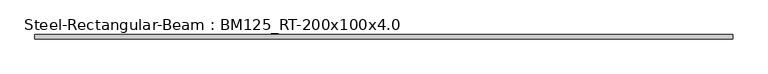
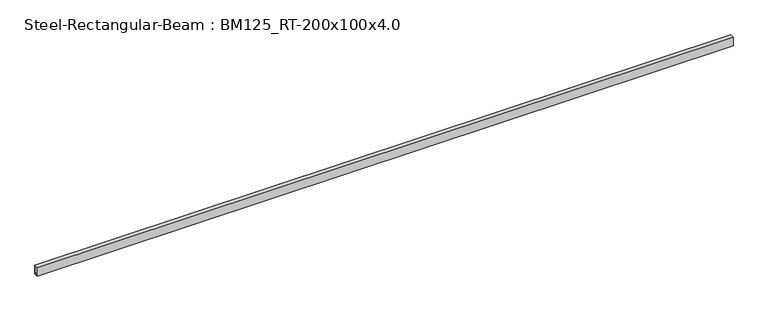
"""IFC4 building model written with IfcOpenShell, lengths in millimetres: beam geometry, Steel-Rectangular-Beam : BM125_RT-200x100x4.0."""

from ifc_helpers import new_model, si_unit, frame, origin, place, context, project, spatial, polyline, outline, extrude, source, transform, mapped, element, save


def steel_rectangular_beam_bm125_rt_200x100x4_0_7795b4bb(model_context):
    return source(origin(), model_context, "Body", "SweptSolid", [
        extrude(outline(polyline([(50.0, 100.0), (50.0, -100.0), (-50.0, -100.0), (-50.0, 100.0), (50.0, 100.0)]), holes=[polyline([(-46.0, -96.0), (46.0, -96.0), (46.0, 96.0), (-46.0, 96.0), (-46.0, -96.0)])]), frame((-8000.0, 0.0, 0.0), z_axis=(1.0, 0.0, 0.0), x_axis=(0.0, 1.0, 0.0)), (0.0, 0.0, 1.0), 16000.0),
        extrude(outline(polyline([(50.0, 100.0), (50.0, -100.0), (-50.0, -100.0), (-50.0, 100.0), (50.0, 100.0)]), holes=[polyline([(-46.0, -96.0), (46.0, -96.0), (46.0, 96.0), (-46.0, 96.0), (-46.0, -96.0)])]), frame((-8000.0, 0.0, 0.0), z_axis=(1.0, 0.0, 0.0), x_axis=(0.0, 1.0, 0.0)), (0.0, 0.0, 1.0), 16000.0),
        extrude(outline(polyline([(50.0, 100.0), (50.0, -100.0), (-50.0, -100.0), (-50.0, 100.0), (50.0, 100.0)]), holes=[polyline([(-46.0, -96.0), (46.0, -96.0), (46.0, 96.0), (-46.0, 96.0), (-46.0, -96.0)])]), frame((-8000.0, 0.0, 0.0), z_axis=(1.0, 0.0, 0.0), x_axis=(0.0, 1.0, 0.0)), (0.0, 0.0, 1.0), 16000.0),
        extrude(outline(polyline([(50.0, 100.0), (50.0, -100.0), (-50.0, -100.0), (-50.0, 100.0), (50.0, 100.0)]), holes=[polyline([(-46.0, -96.0), (46.0, -96.0), (46.0, 96.0), (-46.0, 96.0), (-46.0, -96.0)])]), frame((-8000.0, 0.0, 0.0), z_axis=(1.0, 0.0, 0.0), x_axis=(0.0, 1.0, 0.0)), (0.0, 0.0, 1.0), 16000.0),
    ])


if __name__ == "__main__":
    model = new_model("IFC4")
    model_context = context("Model", 3, world=origin())
    ifc_project = project(units=[si_unit("LENGTHUNIT", "METRE", prefix="MILLI")], contexts=[model_context])
    site = spatial("IfcSite", under=ifc_project)
    building = spatial("IfcBuilding", under=site)
    placement = place(None, origin())
    steel_rectangular_beam_bm125_rt_200x100x4_0_shape = steel_rectangular_beam_bm125_rt_200x100x4_0_7795b4bb(model_context)
    element("IfcBeam", 1, ObjectType="Steel-Rectangular-Beam : BM125_RT-200x100x4.0", at=placement, inside=building, context=model_context, shape_type="MappedRepresentation", body=[
        mapped(steel_rectangular_beam_bm125_rt_200x100x4_0_shape, transform((0.0, 0.0, 0.0), x_axis=(1.0, 0.0, 0.0), y_axis=(0.0, 1.0, 0.0), z_axis=(0.0, 0.0, 1.0))),
    ])
    save(model, "model.ifc")

# Revit data of these elements
# Type "Steel-Rectangular-Beam : BM125_RT-200x100x4.0"
#   t = 4 mm
#   Mass per Unit Length = 18.35 kg/m
#   Surface Area = 0.60 m²/m
#   Sectional Area = 1856.0 cm²
#   Length [instance default] = 3000 mm
#   H = 200 mm
#   B = 100 mm
#   hec_material4 [instance default] = none
#   hec_material3 [instance default] = none
#   hec_material2 [instance default] = none
#   hec_material1 [instance default] = none
#   Structural Material [instance default] = none
# Element 1 (IfcBeam, "Steel-Rectangular-Beam : BM125_RT-200x100x4.0")
#   hec_material2 = S01AA010-00001_Main Steel Structure Fabrication Work_Shelter/Building_Steel Painting/Coating_for Non-Fireproofed Steel Surface, Surface Preparation, Primer, Second & Final Coat
#   hec_material1 = S03AA007-00001_Main Steel Structure Erection Work_Girth & Purlin
#   Structural Material = S01AA007-00001_Main Steel Structure Fabrication Work_Shelter/Building_Girth & Purlin
#   Materials on its faces: "S01AA010-00001_Main Steel Structure Fabrication Work_Shelter/Building_Steel Painting/Coating_for Non-Fireproofed Steel Surface, Surface Preparation, Primer, Second & Final Coat"
# Materials
#   "S01AA010-00001_Main Steel Structure Fabrication Work_Shelter/Building_Steel Painting/Coating_for Non-Fireproofed Steel Surface, Surface Preparation, Primer, Second & Final Coat": class "Metal", colour RGB 120 120 120, transparency 0, Description = "Paint finished steel", W00) Work Master Code = "S01AA010-00001", W01) Work Master_Lv1 = "Main Steel Structure Fabrication Work", W02) Work Master_Lv2 = "Shelter/Building", W03) Work Master_Spec.1 = "Steel Painting/Coating", W04) Work Master_Spec.2 = "for Non-Fireproofed Steel Surface, Surface Preparation, Primer, Second & Final Coat", Cost = 0
#   "S03AA007-00001_Main Steel Structure Erection Work_Girth & Purlin": class "Metal", colour RGB 120 120 120, transparency 0, Comments = "(30KG/M>Weight)", Description = "Structural steel 50ksi", W00) Work Master Code = "S03AA007-00001", W01) Work Master_Lv1 = "Main Steel Structure Erection Work", W02) Work Master_Lv2 = "Shelter/Building", W03) Work Master_Spec.1 = "Girth & Purlin", Cost = 0
#   "S01AA007-00001_Main Steel Structure Fabrication Work_Shelter/Building_Girth & Purlin": class "Metal", colour RGB 120 120 120, transparency 0, Comments = "(30KG/M>Weight)", Description = "Structural steel 50ksi", W00) Work Master Code = "S01AA007-00001", W01) Work Master_Lv1 = "Main Steel Structure Fabrication Work", W02) Work Master_Lv2 = "Shelter/Building", W03) Work Master_Spec.1 = "Girth & Purlin", Cost = 0
